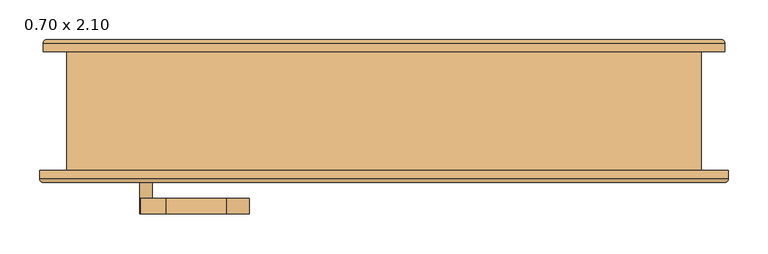
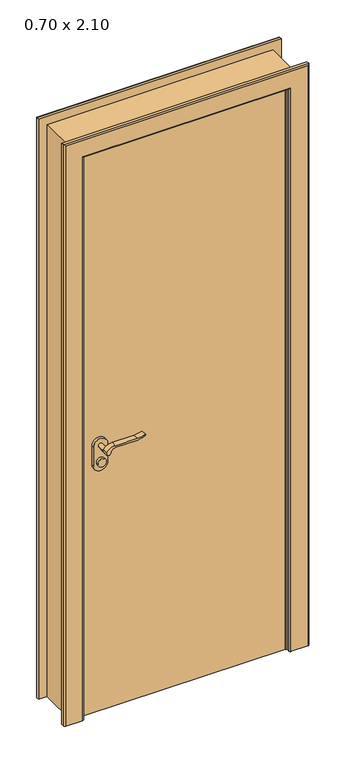
"""IFC4 building model written with IfcOpenShell, lengths in millimetres: door geometry, PORTA_DE_ABRIR_MADEIRA : 0.70 x 2.10."""

from ifc_helpers import new_model, si_unit, point, frame, frame_2d, origin, origin_with_axes, place, context, project, spatial, polyline, circle_curve, ellipse_curve, trimmed, segment, composite_curve, outline, extrude, faceted_brep, source, transform, mapped, element, save
from ifc_brep_helpers import plane_surface, cylinder_surface, advanced_brep


def door_0_70_x_2_10_101532bf(model_context):
    return source(origin(), model_context, "Body", "SolidModel", [
        extrude(outline(composite_curve([segment(trimmed(circle_curve(frame_2d((940.0, -300.0)), 15.0), [point((940.0, -285.0))], [point((940.0, -315.0))], False, "CARTESIAN"), True, "CONTINUOUS"), segment(trimmed(circle_curve(frame_2d((940.0, -300.0)), 15.0), [point((940.0, -315.0))], [point((940.0, -285.0))], False, "CARTESIAN"), True, "CONTINUOUS")], self_intersect=False)), frame((0.0, -25.0, 0.0), z_axis=(0.0, 1.0, 0.0), x_axis=(0.0, 0.0, 1.0)), (0.0, 0.0, 1.0), 10.0),
        extrude(outline(composite_curve([segment(trimmed(circle_curve(frame_2d((940.0, -300.0)), 15.0), [point((940.0, -285.0))], [point((940.0, -315.0))], False, "CARTESIAN"), True, "CONTINUOUS"), segment(trimmed(circle_curve(frame_2d((940.0, -300.0)), 15.0), [point((940.0, -315.0))], [point((940.0, -285.0))], False, "CARTESIAN"), True, "CONTINUOUS")], self_intersect=False)), frame((0.0, -90.0, 0.0), z_axis=(0.0, 1.0, 0.0), x_axis=(0.0, 0.0, 1.0)), (0.0, 0.0, 1.0), 10.0),
        extrude(outline(composite_curve([segment(trimmed(circle_curve(frame_2d((1000.0, -300.0)), 8.0), [point((1004.6523287, -306.5081363))], [point((1000.0, -292.0))], False, "CARTESIAN"), True, "CONTINUOUS"), segment(trimmed(circle_curve(frame_2d((994.8738613, -274.6138099)), 18.1261387), [point((1000.0, -292.0))], [point((1013.0, -274.6138099))], True, "CARTESIAN"), True, "CONTINUOUS"), segment(polyline([(1013.0, -274.6138099), (1013.0, -198.3564091)]), True, "CONTINUOUS"), segment(trimmed(circle_curve(frame_2d((1072.2709207, -201.9396612)), 59.3791355), [point((1013.0, -198.3564091))], [point((1022.2135558, -170.0))], False, "CARTESIAN"), True, "CONTINUOUS"), segment(polyline([(1022.2135558, -170.0), (1025.0, -170.0)]), True, "CONTINUOUS"), segment(trimmed(circle_curve(frame_2d((1103.2850638, -198.4227909)), 83.2850902), [point((1025.0, -170.0))], [point((1020.0, -198.3564091))], True, "CARTESIAN"), True, "CONTINUOUS"), segment(polyline([(1020.0, -198.3564091), (1020.0, -274.6325667)]), True, "CONTINUOUS"), segment(trimmed(circle_curve(frame_2d((982.7555521, -276.3324871)), 37.2832219), [point((1020.0, -274.6325667))], [point((1004.6523287, -306.5081363))], False, "CARTESIAN"), True, "CONTINUOUS")], self_intersect=False)), frame((0.0, 5.0, 0.0), z_axis=(0.0, 1.0, 0.0), x_axis=(0.0, 0.0, 1.0)), (0.0, 0.0, 1.0), 20.0),
        extrude(outline(composite_curve([segment(trimmed(circle_curve(frame_2d((994.8738682, -274.6138122)), 18.1261318), [point((999.9999903, -292.0))], [point((1013.0, -274.6138122))], True, "CARTESIAN"), True, "CONTINUOUS"), segment(polyline([(1013.0, -274.6138122), (1013.0, -198.3564091)]), True, "CONTINUOUS"), segment(trimmed(circle_curve(frame_2d((1072.2709207, -201.9396612)), 59.3791355), [point((1013.0, -198.3564091))], [point((1022.2135558, -170.0))], False, "CARTESIAN"), True, "CONTINUOUS"), segment(polyline([(1022.2135558, -170.0), (1025.0, -170.0)]), True, "CONTINUOUS"), segment(trimmed(circle_curve(frame_2d((1103.2850638, -198.4227909)), 83.2850902), [point((1025.0, -170.0))], [point((1020.0, -198.3564091))], True, "CARTESIAN"), True, "CONTINUOUS"), segment(polyline([(1020.0, -198.3564091), (1020.0, -274.6325667)]), True, "CONTINUOUS"), segment(trimmed(circle_curve(frame_2d((982.7555521, -276.3324871)), 37.2832219), [point((1020.0, -274.6325667))], [point((1004.6523287, -306.5081363))], False, "CARTESIAN"), True, "CONTINUOUS"), segment(trimmed(circle_curve(frame_2d((1000.0, -300.0)), 8.0), [point((1004.6523287, -306.5081363))], [point((999.9999903, -292.0))], False, "CARTESIAN"), True, "CONTINUOUS")], self_intersect=False)), frame((0.0, -130.0, 0.0), z_axis=(0.0, 1.0, 0.0), x_axis=(0.0, 0.0, 1.0)), (0.0, 0.0, 1.0), 20.0),
        extrude(outline(composite_curve([segment(trimmed(circle_curve(frame_2d((1000.0, -300.0)), 8.0), [point((1000.0, -292.0))], [point((1000.0, -308.0))], False, "CARTESIAN"), True, "CONTINUOUS"), segment(trimmed(circle_curve(frame_2d((1000.0, -300.0)), 8.0), [point((1000.0, -308.0))], [point((1000.0, -292.0))], False, "CARTESIAN"), True, "CONTINUOUS")], self_intersect=False)), frame((0.0, -25.0, 0.0), z_axis=(0.0, 1.0, 0.0), x_axis=(0.0, 0.0, 1.0)), (0.0, 0.0, 1.0), 30.0),
        extrude(outline(composite_curve([segment(trimmed(circle_curve(frame_2d((1000.0, -300.0)), 8.0), [point((1000.0, -292.0))], [point((1000.0, -308.0))], False, "CARTESIAN"), True, "CONTINUOUS"), segment(trimmed(circle_curve(frame_2d((1000.0, -300.0)), 8.0), [point((1000.0, -308.0))], [point((1000.0, -292.0))], False, "CARTESIAN"), True, "CONTINUOUS")], self_intersect=False)), frame((0.0, -110.0, 0.0), z_axis=(0.0, 1.0, 0.0), x_axis=(0.0, 0.0, 1.0)), (0.0, 0.0, 1.0), 30.0),
        extrude(outline(composite_curve([segment(trimmed(circle_curve(frame_2d((930.0, -300.0)), 25.0), [point((930.0, -325.0))], [point((930.0, -275.0))], False, "CARTESIAN"), True, "CONTINUOUS"), segment(polyline([(930.0, -275.0), (1000.0, -275.0)]), True, "CONTINUOUS"), segment(trimmed(circle_curve(frame_2d((1000.0, -300.0)), 25.0), [point((1000.0, -275.0))], [point((1000.0, -325.0))], False, "CARTESIAN"), True, "CONTINUOUS"), segment(polyline([(1000.0, -325.0), (930.0, -325.0)]), True, "CONTINUOUS")], self_intersect=False)), frame((0.0, -35.0, 0.0), z_axis=(0.0, 1.0, 0.0), x_axis=(0.0, 0.0, 1.0)), (0.0, 0.0, 1.0), 10.0),
        extrude(outline(composite_curve([segment(trimmed(circle_curve(frame_2d((930.0, -300.0)), 25.0), [point((930.0, -325.0))], [point((930.0, -275.0))], False, "CARTESIAN"), True, "CONTINUOUS"), segment(polyline([(930.0, -275.0), (1000.0, -275.0)]), True, "CONTINUOUS"), segment(trimmed(circle_curve(frame_2d((1000.0, -300.0)), 25.0), [point((1000.0, -275.0))], [point((1000.0, -325.0))], False, "CARTESIAN"), True, "CONTINUOUS"), segment(polyline([(1000.0, -325.0), (930.0, -325.0)]), True, "CONTINUOUS")], self_intersect=False)), frame((0.0, -80.0, 0.0), z_axis=(0.0, 1.0, 0.0), x_axis=(0.0, 0.0, 1.0)), (0.0, 0.0, 1.0), 10.0),
        faceted_brep([(-360.0, -35.0, 0.0), (-360.0, -75.0, 0.0), (-400.0, -75.0, 0.0), (-400.0, 75.0, 0.0), (-350.0, 75.0, 0.0), (-350.0, -35.0, 0.0), (-360.0, -35.0, 2100.0), (-360.0, -75.0, 2100.0), (360.0, -75.0, 2100.0), (360.0, -75.0, 0.0), (400.0, -75.0, 0.0), (400.0, -75.0, 2140.0), (-400.0, -75.0, 2140.0), (-400.0, 75.0, 2140.0), (400.0, 75.0, 2140.0), (400.0, 75.0, 0.0), (350.0, 75.0, 0.0), (350.0, 75.0, 2090.0), (-350.0, 75.0, 2090.0), (-350.0, -35.0, 2090.0), (350.0, -35.0, 2090.0), (350.0, -35.0, 0.0), (360.0, -35.0, 0.0), (360.0, -35.0, 2100.0)], [[[0, 1, 2, 3, 4, 5]], [[1, 0, 6, 7]], [[2, 1, 7, 8, 9, 10, 11, 12]], [[3, 2, 12, 13]], [[4, 3, 13, 14, 15, 16, 17, 18]], [[5, 4, 18, 19]], [[0, 5, 19, 20, 21, 22, 23, 6]], [[20, 17, 16, 21]], [[22, 21, 16, 15, 10, 9]], [[8, 23, 22, 9]], [[14, 11, 10, 15]], [[13, 12, 11, 14]], [[19, 18, 17, 20]], [[7, 6, 23, 8]]]),
        advanced_brep(
        [(-430.0, 75.3, 0.0), (-430.0, 85.3, 0.0), (-425.0, 90.3, 0.0), (-365.0, 90.3, 0.0), (-360.0, 85.3, 0.0), (-360.0, 75.3, 0.0), (-430.0, 75.3, 2170.0), (-430.0, 85.3, 2170.0), (-425.0, 90.3, 2165.0), (425.0, 90.3, 2165.0), (425.0, 90.3, 0.0), (365.0, 90.3, 0.0), (365.0, 90.3, 2105.0), (-365.0, 90.3, 2105.0), (-360.0, 85.3, 2100.0), (-360.0, 75.3, 2100.0), (360.0, 75.3, 2100.0), (360.0, 75.3, 0.0), (430.0, 75.3, 0.0), (430.0, 75.3, 2170.0), (360.0, 85.3, 0.0), (430.0, 85.3, 0.0), (360.0, 85.3, 2100.0), (430.0, 85.3, 2170.0)],
        [
            (0, 1),
            (1, 2, circle_curve(frame((-425.0, 85.3, 0.0), z_axis=(0.0, 0.0, -1.0), x_axis=(-1.0, 0.0, 0.0)), 5.0)),
            (2, 3),
            (3, 4, circle_curve(frame((-365.0, 85.3, 0.0), z_axis=(0.0, 0.0, -1.0), x_axis=(-1.0, 0.0, 0.0)), 5.0)),
            (4, 5),
            (5, 0),
            (0, 6),
            (6, 7),
            (7, 1),
            (7, 8, ellipse_curve(frame((-425.0, 85.3, 2165.0), z_axis=(-0.7071067811865475, 0.0, -0.7071067811865475), x_axis=(0.7071067811865474, 0.0, -0.7071067811865476)), 7.0710678, 5.0)),
            (8, 2),
            (8, 9),
            (9, 10),
            (10, 11),
            (11, 12),
            (12, 13),
            (13, 3),
            (13, 14, ellipse_curve(frame((-365.0, 85.3, 2105.0), z_axis=(-0.7071067811865475, 0.0, -0.7071067811865475), x_axis=(0.7071067811865474, 0.0, -0.7071067811865476)), 7.0710678, 5.0)),
            (14, 4),
            (14, 15),
            (15, 5),
            (15, 16),
            (16, 17),
            (17, 18),
            (18, 19),
            (19, 6),
            (17, 20),
            (20, 11, circle_curve(frame((365.0, 85.3, 0.0), z_axis=(0.0, 0.0, -1.0), x_axis=(1.0, 0.0, 0.0)), 5.0)),
            (10, 21, circle_curve(frame((425.0, 85.3, 0.0), z_axis=(0.0, 0.0, -1.0), x_axis=(1.0, 0.0, 0.0)), 5.0)),
            (21, 18),
            (16, 22),
            (22, 20),
            (22, 12, ellipse_curve(frame((365.0, 85.3, 2105.0), z_axis=(0.7071067811865475, 0.0, -0.7071067811865475), x_axis=(0.7071067811865474, 0.0, 0.7071067811865476)), 7.0710678, 5.0)),
            (9, 23, ellipse_curve(frame((425.0, 85.3, 2165.0), z_axis=(0.7071067811865475, 0.0, -0.7071067811865475), x_axis=(0.7071067811865474, 0.0, 0.7071067811865476)), 7.0710678, 5.0)),
            (23, 21),
            (23, 19),
            (23, 7),
            (14, 22),
        ],
        [
            plane_surface(frame((-400.0, -75.0, 0.0), z_axis=(0.0, 0.0, -1.0), x_axis=(0.0, -1.0, 0.0))),
            plane_surface(frame((-430.0, 75.3, 0.0), z_axis=(-1.0, 0.0, 0.0), x_axis=(0.0, 0.0, 1.0))),
            cylinder_surface(frame((-425.0, 85.3, 0.0), z_axis=(0.0, 0.0, -1.0), x_axis=(-1.0, 0.0, 0.0)), 5.0),
            plane_surface(frame((-425.0, 90.3, 0.0), z_axis=(0.0, 1.0, 0.0), x_axis=(0.0, 0.0, 1.0))),
            cylinder_surface(frame((-365.0, 85.3, 0.0), z_axis=(0.0, 0.0, -1.0), x_axis=(-1.0, 0.0, 0.0)), 5.0),
            plane_surface(frame((-360.0, 85.3, 0.0), z_axis=(1.0, 0.0, 0.0), x_axis=(0.0, 0.0, 1.0))),
            plane_surface(frame((-360.0, 75.3, 0.0), z_axis=(0.0, -1.0, 0.0), x_axis=(0.0, 0.0, 1.0))),
            plane_surface(frame((400.0, -75.0, 0.0), z_axis=(0.0, 0.0, -1.0), x_axis=(0.0, -1.0, 0.0))),
            plane_surface(frame((360.0, 85.3, 2100.0), z_axis=(-1.0, 0.0, 0.0), x_axis=(0.0, 0.0, -1.0))),
            cylinder_surface(frame((365.0, 85.3, 2140.0), z_axis=(0.0, 0.0, 1.0), x_axis=(1.0, 0.0, 0.0)), 5.0),
            cylinder_surface(frame((425.0, 85.3, 2140.0), z_axis=(0.0, 0.0, 1.0), x_axis=(1.0, 0.0, 0.0)), 5.0),
            plane_surface(frame((430.0, 75.3, 2170.0), z_axis=(1.0, 0.0, 0.0), x_axis=(0.0, 0.0, -1.0))),
            plane_surface(frame((-430.0, 75.3, 2170.0), z_axis=(0.0, 0.0, 1.0), x_axis=(1.0, 0.0, 0.0))),
            plane_surface(frame((-360.0, 85.3, 2100.0), z_axis=(0.0, 0.0, -1.0), x_axis=(1.0, 0.0, 0.0))),
            cylinder_surface(frame((-400.0, 85.3, 2165.0), z_axis=(-1.0, 0.0, 0.0), x_axis=(0.0, 0.0, 1.0)), 5.0),
            cylinder_surface(frame((-400.0, 85.3, 2105.0), z_axis=(-1.0, 0.0, 0.0), x_axis=(0.0, 0.0, 1.0)), 5.0),
        ],
        [
            (0, [[1, 2, 3, 4, 5, 6]]),
            (1, [[-1, 7, 8, 9]]),
            (2, [[-2, -9, 10, 11]]),
            (3, [[-3, -11, 12, 13, 14, 15, 16, 17]]),
            (4, [[-4, -17, 18, 19]]),
            (5, [[-5, -19, 20, 21]]),
            (6, [[-6, -21, 22, 23, 24, 25, 26, -7]]),
            (7, [[-24, 27, 28, -14, 29, 30]]),
            (8, [[31, 32, -27, -23]]),
            (9, [[33, -15, -28, -32]]),
            (10, [[34, 35, -29, -13]]),
            (11, [[36, -25, -30, -35]]),
            (12, [[-8, -26, -36, 37]]),
            (13, [[-20, 38, -31, -22]]),
            (14, [[-10, -37, -34, -12]]),
            (15, [[-18, -16, -33, -38]]),
        ],
    ),
        advanced_brep(
        [(-429.3155593, -90.2647517, 0.0), (-434.3155593, -85.2647517, 0.0), (-434.3155593, -75.2647517, 0.0), (-364.3155593, -75.2647517, 0.0), (-364.3155593, -85.2647517, 0.0), (-369.3155593, -90.2647517, 0.0), (-429.3155593, -90.2647517, 2169.3155593), (-434.3155593, -85.2647517, 2174.3155593), (-434.3155593, -75.2647517, 2174.3155593), (434.3155593, -75.2647517, 2174.3155593), (434.3155593, -75.2647517, 0.0), (364.3155593, -75.2647517, 0.0), (364.3155593, -75.2647517, 2104.3155593), (-364.3155593, -75.2647517, 2104.3155593), (-364.3155593, -85.2647517, 2104.3155593), (-369.3155593, -90.2647517, 2109.3155593), (369.3155593, -90.2647517, 2109.3155593), (369.3155593, -90.2647517, 0.0), (429.3155593, -90.2647517, 0.0), (429.3155593, -90.2647517, 2169.3155593), (364.3155593, -85.2647517, 0.0), (434.3155593, -85.2647517, 0.0), (364.3155593, -85.2647517, 2104.3155593), (434.3155593, -85.2647517, 2174.3155593)],
        [
            (0, 1, circle_curve(frame((-429.3155593, -85.2647517, 0.0), z_axis=(0.0, 0.0, -1.0), x_axis=(-1.0, 0.0, 0.0)), 5.0)),
            (1, 2),
            (2, 3),
            (3, 4),
            (4, 5, circle_curve(frame((-369.3155593, -85.2647517, 0.0), z_axis=(0.0, 0.0, -1.0), x_axis=(-1.0, 0.0, 0.0)), 5.0)),
            (5, 0),
            (0, 6),
            (6, 7, ellipse_curve(frame((-429.3155593, -85.2647517, 2169.3155593), z_axis=(-0.7071067811865475, 0.0, -0.7071067811865475), x_axis=(0.7071067811865474, 0.0, -0.7071067811865476)), 7.0710678, 5.0)),
            (7, 1),
            (7, 8),
            (8, 2),
            (8, 9),
            (9, 10),
            (10, 11),
            (11, 12),
            (12, 13),
            (13, 3),
            (13, 14),
            (14, 4),
            (14, 15, ellipse_curve(frame((-369.3155593, -85.2647517, 2109.3155593), z_axis=(-0.7071067811865475, 0.0, -0.7071067811865475), x_axis=(0.7071067811865474, 0.0, -0.7071067811865476)), 7.0710678, 5.0)),
            (15, 5),
            (15, 16),
            (16, 17),
            (17, 18),
            (18, 19),
            (19, 6),
            (17, 20, circle_curve(frame((369.3155593, -85.2647517, 0.0), z_axis=(0.0, 0.0, -1.0), x_axis=(1.0, 0.0, 0.0)), 5.0)),
            (20, 11),
            (10, 21),
            (21, 18, circle_curve(frame((429.3155593, -85.2647517, 0.0), z_axis=(0.0, 0.0, -1.0), x_axis=(1.0, 0.0, 0.0)), 5.0)),
            (16, 22, ellipse_curve(frame((369.3155593, -85.2647517, 2109.3155593), z_axis=(0.7071067811865475, 0.0, -0.7071067811865475), x_axis=(0.7071067811865474, 0.0, 0.7071067811865476)), 7.0710678, 5.0)),
            (22, 20),
            (22, 12),
            (9, 23),
            (23, 21),
            (23, 19, ellipse_curve(frame((429.3155593, -85.2647517, 2169.3155593), z_axis=(0.7071067811865475, 0.0, -0.7071067811865475), x_axis=(0.7071067811865474, 0.0, 0.7071067811865476)), 7.0710678, 5.0)),
            (7, 23),
            (22, 14),
        ],
        [
            plane_surface(frame((-400.0, -75.0, 0.0), z_axis=(0.0, 0.0, -1.0), x_axis=(0.0, -1.0, 0.0))),
            cylinder_surface(frame((-429.3155593, -85.2647517, 0.0), z_axis=(0.0, 0.0, -1.0), x_axis=(-1.0, 0.0, 0.0)), 5.0),
            plane_surface(frame((-434.3155593, -85.2647517, 0.0), z_axis=(-1.0, 0.0, 0.0), x_axis=(0.0, 0.0, 1.0))),
            plane_surface(frame((-434.3155593, -75.2647517, 0.0), z_axis=(0.0, 1.0, 0.0), x_axis=(0.0, 0.0, 1.0))),
            plane_surface(frame((-364.3155593, -75.2647517, 0.0), z_axis=(1.0, 0.0, 0.0), x_axis=(0.0, 0.0, 1.0))),
            cylinder_surface(frame((-369.3155593, -85.2647517, 0.0), z_axis=(0.0, 0.0, -1.0), x_axis=(-1.0, 0.0, 0.0)), 5.0),
            plane_surface(frame((-369.3155593, -90.2647517, 0.0), z_axis=(0.0, -1.0, 0.0), x_axis=(0.0, 0.0, 1.0))),
            plane_surface(frame((400.0, -75.0, 0.0), z_axis=(0.0, 0.0, -1.0), x_axis=(0.0, -1.0, 0.0))),
            cylinder_surface(frame((369.3155593, -85.2647517, 2140.0), z_axis=(0.0, 0.0, 1.0), x_axis=(1.0, 0.0, 0.0)), 5.0),
            plane_surface(frame((364.3155593, -75.2647517, 2104.3155593), z_axis=(-1.0, 0.0, 0.0), x_axis=(0.0, 0.0, -1.0))),
            plane_surface(frame((434.3155593, -85.2647517, 2174.3155593), z_axis=(1.0, 0.0, 0.0), x_axis=(0.0, 0.0, -1.0))),
            cylinder_surface(frame((429.3155593, -85.2647517, 2140.0), z_axis=(0.0, 0.0, 1.0), x_axis=(1.0, 0.0, 0.0)), 5.0),
            plane_surface(frame((-434.3155593, -85.2647517, 2174.3155593), z_axis=(0.0, 0.0, 1.0), x_axis=(1.0, 0.0, 0.0))),
            plane_surface(frame((-364.3155593, -75.2647517, 2104.3155593), z_axis=(0.0, 0.0, -1.0), x_axis=(1.0, 0.0, 0.0))),
            cylinder_surface(frame((-400.0, -85.2647517, 2169.3155593), z_axis=(-1.0, 0.0, 0.0), x_axis=(0.0, 0.0, 1.0)), 5.0),
            cylinder_surface(frame((-400.0, -85.2647517, 2109.3155593), z_axis=(-1.0, 0.0, 0.0), x_axis=(0.0, 0.0, 1.0)), 5.0),
        ],
        [
            (0, [[1, 2, 3, 4, 5, 6]]),
            (1, [[-1, 7, 8, 9]]),
            (2, [[-2, -9, 10, 11]]),
            (3, [[-3, -11, 12, 13, 14, 15, 16, 17]]),
            (4, [[-4, -17, 18, 19]]),
            (5, [[-5, -19, 20, 21]]),
            (6, [[-6, -21, 22, 23, 24, 25, 26, -7]]),
            (7, [[-24, 27, 28, -14, 29, 30]]),
            (8, [[31, 32, -27, -23]]),
            (9, [[33, -15, -28, -32]]),
            (10, [[34, 35, -29, -13]]),
            (11, [[36, -25, -30, -35]]),
            (12, [[-10, 37, -34, -12]]),
            (13, [[-18, -16, -33, 38]]),
            (14, [[-8, -26, -36, -37]]),
            (15, [[-20, -38, -31, -22]]),
        ],
    ),
        extrude(outline(polyline([(360.0, -70.0), (-360.0, -70.0), (-360.0, -35.0), (360.0, -35.0), (360.0, -70.0)])), origin_with_axes(), (0.0, 0.0, 1.0), 2100.0),
    ])


if __name__ == "__main__":
    model = new_model("IFC4")
    model_context = context("Model", 3, world=origin())
    ifc_project = project(units=[si_unit("LENGTHUNIT", "METRE", prefix="MILLI")], contexts=[model_context])
    site = spatial("IfcSite", under=ifc_project)
    building = spatial("IfcBuilding", under=site)
    placement = place(None, origin())
    door_0_70_x_2_10_shape = door_0_70_x_2_10_101532bf(model_context)
    element("IfcDoor", 1, ObjectType="PORTA_DE_ABRIR_MADEIRA : 0.70 x 2.10", at=placement, inside=building, context=model_context, shape_type="MappedRepresentation", body=[
        mapped(door_0_70_x_2_10_shape, transform((0.0, 0.0, 0.0), x_axis=(1.0, 0.0, 0.0), y_axis=(0.0, 1.0, 0.0), z_axis=(0.0, 0.0, 1.0))),
    ])
    save(model, "model.ifc")

# Revit data of these elements
# Type "PORTA_DE_ABRIR_MADEIRA : 0.70 x 2.10"
#   Type Mark = "P3"
#   Analytic Construction = "<Nenhum>"
#   Rough Width = 0.80 m
#   Projeção da estrutura externa = 0.025 m
#   Projeção da estrutura interna = 0.025 m
#   Largura da estrutura = 0.075 m
#   Rough Height = 2.15 m
#   Height = 2.10 m
#   Width = 0.70 m
#   Soleira [instance default] = no
#   Material do batente = .BATENTE E GUARNIÇÃO
#   Material da maçaneta = .AÇO INOXIDÁVEL ESCOVADO
#   Material da folha da porta = .FOLHA DA PORTA
#   Material da Soleira [instance default] = none
#   Function = (empty or 0)
#   Wall Closure = (empty or 0)
# Element 1 (IfcDoor, "PORTA_DE_ABRIR_MADEIRA : 0.70 x 2.10")
#   Materials on its faces: ".AÇO INOXIDÁVEL ESCOVADO", ".BATENTE E GUARNIÇÃO", ".FOLHA DA PORTA"
# Materials
#   ".BATENTE E GUARNIÇÃO": class "Madeira", colour RGB 215 186 156, transparency 0, Cost = 0
#   ".AÇO INOXIDÁVEL ESCOVADO": class "Metal", colour RGB 189 187 185, transparency 0, Description = "Stainless Steel 18/8, brushed finish", Cost = 0
#   ".FOLHA DA PORTA": class "Madeira", colour RGB 148 119 91, transparency 0, Cost = 0
